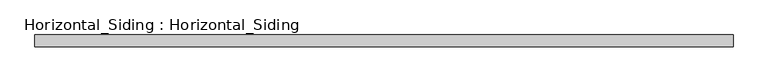
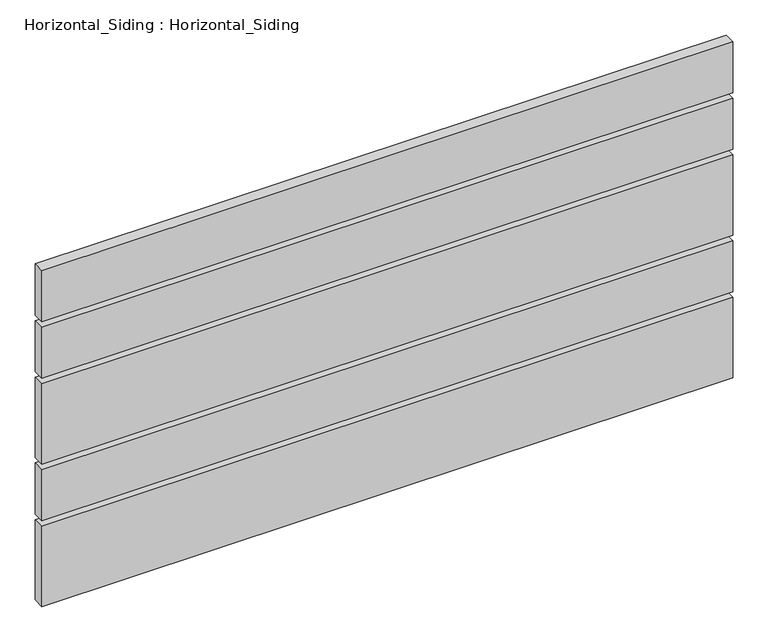
"""IFC4 building model written with IfcOpenShell, lengths in millimetres: plate geometry, Horizontal_Siding : Horizontal_Siding."""

from ifc_helpers import new_model, si_unit, frame, origin, place, context, project, spatial, polyline, outline, extrude, source, transform, mapped, element, save


def horizontal_siding_horizontal_siding_3c0b2188(model_context):
    return source(origin(), model_context, "Body", "SweptSolid", [
        extrude(outline(polyline([(568.325, -19.05), (-568.325, -19.05), (-568.325, 0.0), (568.325, 0.0), (568.325, -19.05)])), frame((0.0, 0.0, 9.525), z_axis=(0.0, 0.0, 1.0), x_axis=(1.0, 0.0, 0.0)), (0.0, 0.0, 1.0), 139.7),
        extrude(outline(polyline([(568.325, -19.05), (-568.325, -19.05), (-568.325, 0.0), (568.325, 0.0), (568.325, -19.05)])), frame((0.0, 0.0, 158.75), z_axis=(0.0, 0.0, 1.0), x_axis=(1.0, 0.0, 0.0)), (0.0, 0.0, 1.0), 88.9),
        extrude(outline(polyline([(568.325, -19.05), (-568.325, -19.05), (-568.325, 0.0), (568.325, 0.0), (568.325, -19.05)])), frame((0.0, 0.0, 257.175), z_axis=(0.0, 0.0, 1.0), x_axis=(1.0, 0.0, 0.0)), (0.0, 0.0, 1.0), 139.7),
        extrude(outline(polyline([(568.325, -19.05), (-568.325, -19.05), (-568.325, 0.0), (568.325, 0.0), (568.325, -19.05)])), frame((0.0, 0.0, 406.4), z_axis=(0.0, 0.0, 1.0), x_axis=(1.0, 0.0, 0.0)), (0.0, 0.0, 1.0), 88.9),
        extrude(outline(polyline([(568.325, -19.05), (-568.325, -19.05), (-568.325, 0.0), (568.325, 0.0), (568.325, -19.05)])), frame((0.0, 0.0, 504.825), z_axis=(0.0, 0.0, 1.0), x_axis=(1.0, 0.0, 0.0)), (0.0, 0.0, 1.0), 88.9),
    ])


if __name__ == "__main__":
    model = new_model("IFC4")
    model_context = context("Model", 3, world=origin())
    ifc_project = project(units=[si_unit("LENGTHUNIT", "METRE", prefix="MILLI")], contexts=[model_context])
    site = spatial("IfcSite", under=ifc_project)
    building = spatial("IfcBuilding", under=site)
    placement = place(None, origin())
    horizontal_siding_horizontal_siding_shape = horizontal_siding_horizontal_siding_3c0b2188(model_context)
    element("IfcPlate", 1, ObjectType="Horizontal_Siding : Horizontal_Siding", at=placement, inside=building, context=model_context, shape_type="MappedRepresentation", body=[
        mapped(horizontal_siding_horizontal_siding_shape, transform((0.0, 0.0, 0.0), x_axis=(1.0, 0.0, 0.0), y_axis=(0.0, 1.0, 0.0), z_axis=(0.0, 0.0, 1.0))),
    ])
    save(model, "model.ifc")

# Revit data of these elements
# Type "Horizontal_Siding : Horizontal_Siding"
#   Analytic Construction = "<None>"
#   extend = 0' - 2 3/4"
#   Width_2 = 0' - 3 1/2"
#   Width_1 = 0' - 5 1/2"
#   Gap = 0' - 0 3/8"
#   Plank Material = SLOTTED WOOD FENCE (THERMALLY MODIFIED WOOD: ARBOR WOOD)\n(EXTERIOR STAIN : PENOFIN VERDE EXT. STAIN - COLOR: CEDAR)
# Element 1 (IfcPlate, "Horizontal_Siding : Horizontal_Siding")
#   Materials on its faces: "SLOTTED WOOD FENCE (THERMALLY MODIFIED WOOD: ARBOR WOOD)\n(EXTERIOR STAIN : PENOFIN VERDE EXT. STAIN - COLOR: CEDAR)"
# Materials
#   "SLOTTED WOOD FENCE (THERMALLY MODIFIED WOOD: ARBOR WOOD)\n(EXTERIOR STAIN : PENOFIN VERDE EXT. STAIN - COLOR: CEDAR)": class "Wood", colour RGB 164 134 123, transparency 0, Description = "Pinus Echinata", Cost = 0
